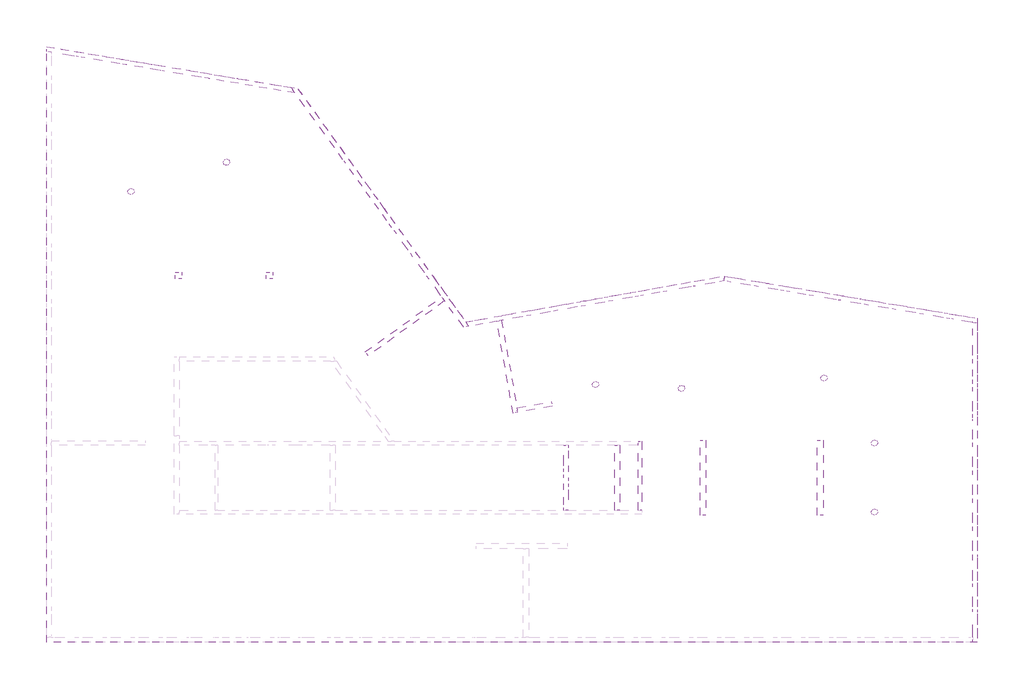
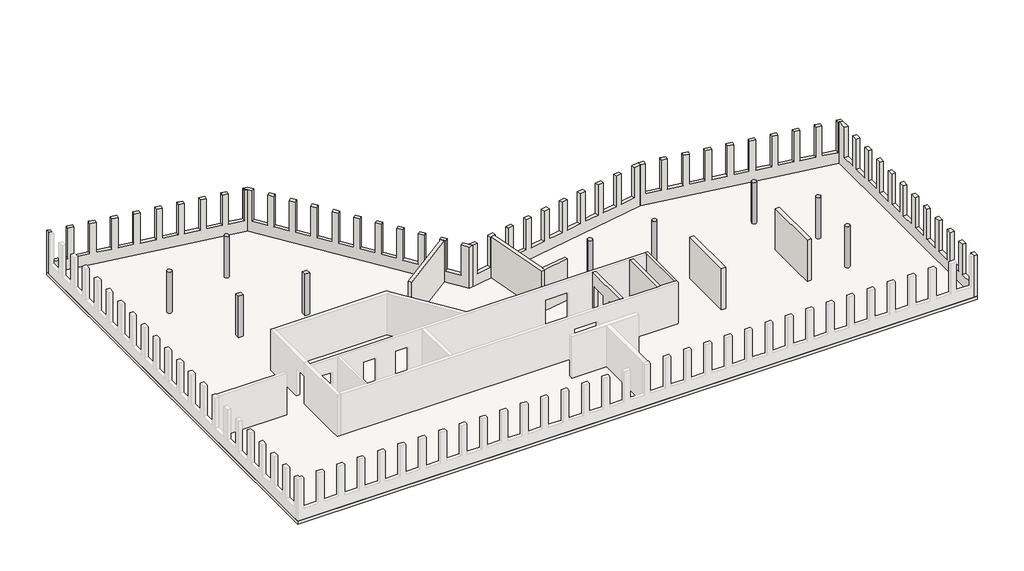
# One storey, part 2 of 2: 13 walls, 9 columns, 1 slab.
"""IFC4 building model written with IfcOpenShell, lengths in millimetres."""

from ifc_helpers import new_model, si_unit, point, frame, frame_2d, origin, place, context, project, spatial, polyline, circle_curve, trimmed, segment, composite_curve, outline, extrude, faceted_brep, element, save

model = new_model("IFC4")

# Units and contexts
model_context = context("Model", 3, world=origin())
ifc_project = project(units=[si_unit("LENGTHUNIT", "METRE", prefix="MILLI")], contexts=[model_context])

# Site, building, storey
site = spatial("IfcSite", under=ifc_project)
building = spatial("IfcBuilding", under=site)
storey = spatial("IfcBuildingStorey", under=building, Name="01_OG_OKFB_3,46", Elevation=3460.0)

# Columns
placement = place(None, origin())
element("IfcColumn", 1, ObjectType="5dki STB-Stützen rund : 5dki Stütze rund ø35cm C40/50", at=placement, inside=storey, context=model_context, shape_type="SweptSolid", body=[
    extrude(outline(composite_curve([segment(trimmed(circle_curve(frame_2d((33961.7583834, 13503.0230367)), 175.0), [point((34136.7583834, 13503.0230367))], [point((33786.7583834, 13503.0230367))], False, "CARTESIAN"), True, "CONTINUOUS"), segment(trimmed(circle_curve(frame_2d((33961.7583834, 13503.0230367)), 175.0), [point((33786.7583834, 13503.0230367))], [point((34136.7583834, 13503.0230367))], False, "CARTESIAN"), True, "CONTINUOUS")], self_intersect=False)), frame((0.0, 0.0, 6770.0), z_axis=(0.0, 0.0, 1.0), x_axis=(1.0, 0.0, 0.0)), (0.0, 0.0, 1.0), 3210.0),
])
element("IfcColumn", 2, ObjectType="5dki STB-Stützen rechteckig : 5dki Stütze recht. 35x35cm C35/45", at=placement, inside=storey, context=model_context, shape_type="SweptSolid", body=[
    extrude(outline(polyline([(7139.9999521, 19742.0124565), (7139.9999521, 19392.0124565), (6789.9999521, 19392.0124565), (6789.9999521, 19742.0124565), (7139.9999521, 19742.0124565)])), frame((0.0, 0.0, 6770.0), z_axis=(0.0, 0.0, 1.0), x_axis=(1.0, 0.0, 0.0)), (0.0, 0.0, 1.0), 3210.0),
])
element("IfcColumn", 3, ObjectType="5dki STB-Stützen rechteckig : 5dki Stütze recht. 35x35cm C35/45", at=placement, inside=storey, context=model_context, shape_type="SweptSolid", body=[
    extrude(outline(polyline([(12021.4450432, 19742.0124565), (12021.4450432, 19392.0124565), (11671.4450432, 19392.0124565), (11671.4450432, 19742.0124565), (12021.4450432, 19742.0124565)])), frame((0.0, 0.0, 6770.0), z_axis=(0.0, 0.0, 1.0), x_axis=(1.0, 0.0, 0.0)), (0.0, 0.0, 1.0), 3210.0),
])
element("IfcColumn", 4, ObjectType="5dki STB-Stützen rund : 5dki Stütze rund ø35cm C40/50", at=placement, inside=storey, context=model_context, shape_type="SweptSolid", body=[
    extrude(outline(composite_curve([segment(trimmed(circle_curve(frame_2d((41616.0718251, 14052.9332427)), 175.0), [point((41791.0718251, 14052.9332427))], [point((41441.0718251, 14052.9332427))], False, "CARTESIAN"), True, "CONTINUOUS"), segment(trimmed(circle_curve(frame_2d((41616.0718251, 14052.9332427)), 175.0), [point((41441.0718251, 14052.9332427))], [point((41791.0718251, 14052.9332427))], False, "CARTESIAN"), True, "CONTINUOUS")], self_intersect=False)), frame((0.0, 0.0, 6770.0), z_axis=(0.0, 0.0, 1.0), x_axis=(1.0, 0.0, 0.0)), (0.0, 0.0, 1.0), 3210.0),
])
element("IfcColumn", 5, ObjectType="5dki STB-Stützen rund : 5dki Stütze rund ø35cm C40/50", at=placement, inside=storey, context=model_context, shape_type="SweptSolid", body=[
    extrude(outline(composite_curve([segment(trimmed(circle_curve(frame_2d((44328.9990923, 10566.8309986)), 175.0), [point((44503.9990923, 10566.8309986))], [point((44153.9990923, 10566.8309986))], False, "CARTESIAN"), True, "CONTINUOUS"), segment(trimmed(circle_curve(frame_2d((44328.9990923, 10566.8309986)), 175.0), [point((44153.9990923, 10566.8309986))], [point((44503.9990923, 10566.8309986))], False, "CARTESIAN"), True, "CONTINUOUS")], self_intersect=False)), frame((0.0, 0.0, 6770.0), z_axis=(0.0, 0.0, 1.0), x_axis=(1.0, 0.0, 0.0)), (0.0, 0.0, 1.0), 3210.0),
])
element("IfcColumn", 6, ObjectType="5dki STB-Stützen rund : 5dki Stütze rund ø35cm C40/50", at=placement, inside=storey, context=model_context, shape_type="SweptSolid", body=[
    extrude(outline(composite_curve([segment(trimmed(circle_curve(frame_2d((44328.9990923, 6852.1619165)), 175.0), [point((44503.9990923, 6852.1619165))], [point((44153.9990923, 6852.1619165))], False, "CARTESIAN"), True, "CONTINUOUS"), segment(trimmed(circle_curve(frame_2d((44328.9990923, 6852.1619165)), 175.0), [point((44153.9990923, 6852.1619165))], [point((44503.9990923, 6852.1619165))], False, "CARTESIAN"), True, "CONTINUOUS")], self_intersect=False)), frame((0.0, 0.0, 6770.0), z_axis=(0.0, 0.0, 1.0), x_axis=(1.0, 0.0, 0.0)), (0.0, 0.0, 1.0), 3210.0),
])
element("IfcColumn", 7, ObjectType="5dki STB-Stützen rund : 5dki Stütze rund ø35cm C40/50", at=placement, inside=storey, context=model_context, shape_type="SweptSolid", body=[
    extrude(outline(composite_curve([segment(trimmed(circle_curve(frame_2d((9535.2710874, 25643.9282611)), 175.0), [point((9710.2710874, 25643.9282611))], [point((9360.2710874, 25643.9282611))], False, "CARTESIAN"), True, "CONTINUOUS"), segment(trimmed(circle_curve(frame_2d((9535.2710874, 25643.9282611)), 175.0), [point((9360.2710874, 25643.9282611))], [point((9710.2710874, 25643.9282611))], False, "CARTESIAN"), True, "CONTINUOUS")], self_intersect=False)), frame((0.0, 0.0, 6770.0), z_axis=(0.0, 0.0, 1.0), x_axis=(1.0, 0.0, 0.0)), (0.0, 0.0, 1.0), 3210.0),
])
element("IfcColumn", 8, ObjectType="5dki STB-Stützen rund : 5dki Stütze rund ø35cm C40/50", at=placement, inside=storey, context=model_context, shape_type="SweptSolid", body=[
    extrude(outline(composite_curve([segment(trimmed(circle_curve(frame_2d((4404.9034618, 24066.2757931)), 175.0), [point((4579.9034618, 24066.2757931))], [point((4229.9034618, 24066.2757931))], False, "CARTESIAN"), True, "CONTINUOUS"), segment(trimmed(circle_curve(frame_2d((4404.9034618, 24066.2757931)), 175.0), [point((4229.9034618, 24066.2757931))], [point((4579.9034618, 24066.2757931))], False, "CARTESIAN"), True, "CONTINUOUS")], self_intersect=False)), frame((0.0, 0.0, 6770.0), z_axis=(0.0, 0.0, 1.0), x_axis=(1.0, 0.0, 0.0)), (0.0, 0.0, 1.0), 3210.0),
])
element("IfcColumn", 9, ObjectType="5dki STB-Stützen rund : 5dki Stütze rund ø35cm C40/50", at=placement, inside=storey, context=model_context, shape_type="SweptSolid", body=[
    extrude(outline(composite_curve([segment(trimmed(circle_curve(frame_2d((29357.7423112, 13702.251654)), 175.0), [point((29532.7423112, 13702.251654))], [point((29182.7423112, 13702.251654))], False, "CARTESIAN"), True, "CONTINUOUS"), segment(trimmed(circle_curve(frame_2d((29357.7423112, 13702.251654)), 175.0), [point((29182.7423112, 13702.251654))], [point((29532.7423112, 13702.251654))], False, "CARTESIAN"), True, "CONTINUOUS")], self_intersect=False)), frame((0.0, 0.0, 6770.0), z_axis=(0.0, 0.0, 1.0), x_axis=(1.0, 0.0, 0.0)), (0.0, 0.0, 1.0), 3210.0),
])

# Slab
element("IfcSlab", 10, ObjectType="5dki Decke Ortbeton 25cm C30/37", at=placement, inside=storey, context=model_context, shape_type="SweptSolid", body=[
    extrude(outline(polyline([(-129.9989953, 31855.7150729), (13359.8955383, 29603.0549033), (22383.5041721, 17069.4128529), (36259.9888873, 19532.5499737), (49863.9990833, 17260.8337794), (49863.9991105, -129.9989509), (-129.9989953, -129.9990284), (-129.9989953, 31855.7150729)]), holes=[polyline([(30391.9999891, 10442.0127433), (27891.9999829, 10442.0127433), (27891.9999829, 6960.0000498), (30391.9999891, 6960.0000498), (30391.9999891, 10442.0127433)]), polyline([(31641.9999382, 10442.0127483), (30641.9999891, 10442.0127483), (30641.9999891, 6960.0000514), (31641.9999382, 6960.0000514), (31641.9999382, 10442.0127483)]), polyline([(8916.9999886, 10442.0127052), (6989.9995723, 10442.0127052), (6989.9995723, 6960.0000232), (8916.9999886, 6960.0000232), (8916.9999886, 10442.0127052)]), polyline([(24127.0004657, 8820.0328918), (16927.0004692, 8820.0328918), (16927.0004692, 7020.033352), (24127.0004657, 7020.033352), (24127.0004657, 8820.0328918)])]), frame((0.0, 0.0, 6520.0), z_axis=(0.0, 0.0, 1.0), x_axis=(1.0, 0.0, 0.0)), (0.0, 0.0, 1.0), 250.0),
])

# Walls
element("IfcWall", 11, ObjectType="5dki Lochfassade 26cm C30/37", at=placement, inside=storey, context=model_context, shape_type="Brep", body=[
    faceted_brep([(12995.7423601, 29663.864375, 6770.0), (13211.4553837, 29364.2425792, 6770.0), (22268.004401, 16784.8468851, 6770.0), (22268.004401, 16784.8468851, 9980.0), (21924.4906268, 17261.9817942, 9980.0), (21924.4906268, 17261.9817942, 7630.0), (21293.4697845, 18138.4592307, 7630.0), (21293.4697845, 18138.4592307, 9980.0), (21048.0727903, 18479.3115671, 9980.0), (21048.0727903, 18479.3115671, 7630.0), (20417.0519481, 19355.7890035, 7630.0), (20417.0519481, 19355.7890035, 9980.0), (20171.6549538, 19696.64134, 9980.0), (20171.6549538, 19696.64134, 7630.0), (19540.6341116, 20573.1187764, 7630.0), (19540.6341116, 20573.1187764, 9980.0), (19295.2371174, 20913.9711128, 9980.0), (19295.2371174, 20913.9711128, 7630.0), (18664.2162751, 21790.4485493, 7630.0), (18664.2162751, 21790.4485493, 9980.0), (18418.8192809, 22131.3008857, 9980.0), (18418.8192809, 22131.3008857, 7630.0), (17787.7984387, 23007.7783222, 7630.0), (17787.7984387, 23007.7783222, 9980.0), (17542.4014445, 23348.6306586, 9980.0), (17542.4014445, 23348.6306586, 7630.0), (16911.3806022, 24225.1080951, 7630.0), (16911.3806022, 24225.1080951, 9980.0), (16665.983608, 24565.9604315, 9980.0), (16665.983608, 24565.9604315, 7630.0), (16034.9627658, 25442.4378679, 7630.0), (16034.9627658, 25442.4378679, 9980.0), (15789.5657715, 25783.2902043, 9980.0), (15789.5657715, 25783.2902043, 7630.0), (15158.5449293, 26659.7676408, 7630.0), (15158.5449293, 26659.7676408, 9980.0), (14913.1479351, 27000.6199772, 9980.0), (14913.1479351, 27000.6199772, 7630.0), (14282.1270928, 27877.0974137, 7630.0), (14282.1270928, 27877.0974137, 9980.0), (14036.7300986, 28217.9497501, 9980.0), (14036.7300986, 28217.9497501, 7630.0), (13405.7092564, 29094.4271866, 7630.0), (13405.7092564, 29094.4271866, 9980.0), (13211.4553837, 29364.2425792, 9980.0), (13028.1664453, 29618.8278609, 9980.0), (13028.1664453, 29618.8278609, 7630.0), (12995.7423601, 29663.864375, 7630.0), (22552.0750732, 16835.2706799, 6770.0), (22383.5041721, 17069.4128529, 6770.0), (13359.8955383, 29603.0549033, 6770.0), (13359.8955383, 29603.0549033, 9980.0), (13616.7130837, 29246.3396115, 9980.0), (13616.7130837, 29246.3396115, 7630.0), (14247.7339259, 28369.8621751, 7630.0), (14247.7339259, 28369.8621751, 9980.0), (14493.1309201, 28029.0098387, 9980.0), (14493.1309201, 28029.0098387, 7630.0), (15124.1517624, 27152.5324022, 7630.0), (15124.1517624, 27152.5324022, 9980.0), (15369.5487566, 26811.6800658, 9980.0), (15369.5487566, 26811.6800658, 7630.0), (16000.5695988, 25935.2026293, 7630.0), (16000.5695988, 25935.2026293, 9980.0), (16245.966593, 25594.3502929, 9980.0), (16245.966593, 25594.3502929, 7630.0), (16876.9874353, 24717.8728564, 7630.0), (16876.9874353, 24717.8728564, 9980.0), (17122.3844295, 24377.02052, 9980.0), (17122.3844295, 24377.02052, 7630.0), (17753.4052718, 23500.5430836, 7630.0), (17753.4052718, 23500.5430836, 9980.0), (17998.802266, 23159.6907472, 9980.0), (17998.802266, 23159.6907472, 7630.0), (18629.8231082, 22283.2133107, 7630.0), (18629.8231082, 22283.2133107, 9980.0), (18875.2201024, 21942.3609743, 9980.0), (18875.2201024, 21942.3609743, 7630.0), (19506.2409447, 21065.8835378, 7630.0), (19506.2409447, 21065.8835378, 9980.0), (19751.6379389, 20725.0312014, 9980.0), (19751.6379389, 20725.0312014, 7630.0), (20382.6587811, 19848.5537649, 7630.0), (20382.6587811, 19848.5537649, 9980.0), (20628.0557754, 19507.7014285, 9980.0), (20628.0557754, 19507.7014285, 7630.0), (21259.0766176, 18631.2239921, 7630.0), (21259.0766176, 18631.2239921, 9980.0), (21504.4736118, 18290.3716557, 9980.0), (21504.4736118, 18290.3716557, 7630.0), (22135.4944541, 17413.8942192, 7630.0), (22135.4944541, 17413.8942192, 9980.0), (22383.5041721, 17069.4128529, 9980.0), (22552.0750732, 16835.2706799, 9980.0), (13034.6033862, 29657.3750221, 9980.0), (13034.6033862, 29657.3750221, 7630.0)], [[[0, 1, 2, 3, 4, 5, 6, 7, 8, 9, 10, 11, 12, 13, 14, 15, 16, 17, 18, 19, 20, 21, 22, 23, 24, 25, 26, 27, 28, 29, 30, 31, 32, 33, 34, 35, 36, 37, 38, 39, 40, 41, 42, 43, 44, 45, 46, 47]], [[48, 49, 50, 51, 52, 53, 54, 55, 56, 57, 58, 59, 60, 61, 62, 63, 64, 65, 66, 67, 68, 69, 70, 71, 72, 73, 74, 75, 76, 77, 78, 79, 80, 81, 82, 83, 84, 85, 86, 87, 88, 89, 90, 91, 92, 93]], [[2, 1, 0, 50, 49, 48]], [[3, 93, 92, 91, 4]], [[52, 51, 94, 45, 44, 43]], [[55, 40, 39, 56]], [[59, 36, 35, 60]], [[63, 32, 31, 64]], [[67, 28, 27, 68]], [[71, 24, 23, 72]], [[75, 20, 19, 76]], [[79, 16, 15, 80]], [[83, 12, 11, 84]], [[87, 8, 7, 88]], [[3, 2, 48, 93]], [[42, 53, 52, 43]], [[54, 41, 40, 55]], [[53, 42, 41, 54]], [[39, 38, 57, 56]], [[37, 36, 59, 58]], [[38, 37, 58, 57]], [[35, 34, 61, 60]], [[33, 32, 63, 62]], [[34, 33, 62, 61]], [[31, 30, 65, 64]], [[29, 28, 67, 66]], [[30, 29, 66, 65]], [[27, 26, 69, 68]], [[25, 24, 71, 70]], [[26, 25, 70, 69]], [[23, 22, 73, 72]], [[21, 20, 75, 74]], [[22, 21, 74, 73]], [[19, 18, 77, 76]], [[17, 16, 79, 78]], [[18, 17, 78, 77]], [[15, 14, 81, 80]], [[13, 12, 83, 82]], [[14, 13, 82, 81]], [[11, 10, 85, 84]], [[9, 8, 87, 86]], [[10, 9, 86, 85]], [[7, 6, 89, 88]], [[5, 4, 91, 90]], [[6, 5, 90, 89]], [[51, 50, 0, 47, 95, 94]], [[95, 46, 45, 94]], [[46, 95, 47]]]),
])
element("IfcWall", 12, ObjectType="5dki Lochfassade 26cm C30/37", at=placement, inside=storey, context=model_context, shape_type="Brep", body=[
    faceted_brep([(27318.6765704, 17681.3634281, 9980.0), (26924.8330267, 17611.4544654, 9980.0), (26924.8330267, 17611.4544654, 7630.0), (25861.4554587, 17422.7002661, 7630.0), (25861.4554587, 17422.7002661, 9980.0), (25447.9197377, 17349.2958553, 9980.0), (25447.9197377, 17349.2958553, 7630.0), (24384.5421697, 17160.541656, 7630.0), (24384.5421697, 17160.541656, 9980.0), (24300.8505369, 17145.6860228, 9980.0), (24054.698322, 17101.9929211, 9980.0), (23971.0064488, 17087.1372452, 9980.0), (23971.0064488, 17087.1372452, 7630.0), (22907.6288807, 16898.3830459, 7630.0), (22907.6288807, 16898.3830459, 9980.0), (22552.0750732, 16835.2706799, 9980.0), (22552.0750732, 16835.2706799, 6770.0), (24054.698322, 17101.9929211, 6770.0), (24300.8505369, 17145.6860228, 6770.0), (36261.33607, 19268.7248546, 6770.0), (36261.33607, 19268.7248546, 9980.0), (35766.6205834, 19180.910678, 9980.0), (35766.6205834, 19180.910678, 7630.0), (34703.2430153, 18992.1564787, 7630.0), (34703.2430153, 18992.1564787, 9980.0), (34289.7072944, 18918.7520679, 9980.0), (34289.7072944, 18918.7520679, 7630.0), (33226.3297263, 18729.9978686, 7630.0), (33226.3297263, 18729.9978686, 9980.0), (32812.7940054, 18656.5934577, 9980.0), (32812.7940054, 18656.5934577, 7630.0), (31749.4164374, 18467.8392585, 7630.0), (31749.4164374, 18467.8392585, 9980.0), (31335.8807164, 18394.4348476, 9980.0), (31335.8807164, 18394.4348476, 7630.0), (30272.5031484, 18205.6806483, 7630.0), (30272.5031484, 18205.6806483, 9980.0), (29858.9674275, 18132.2762375, 9980.0), (29858.9674275, 18132.2762375, 7630.0), (28795.5898594, 17943.5220382, 7630.0), (28795.5898594, 17943.5220382, 9980.0), (28382.0541385, 17870.1176274, 9980.0), (28382.0541385, 17870.1176274, 7630.0), (27318.6765704, 17681.3634281, 7630.0), (26879.392201, 17867.4527688, 7630.0), (26879.392201, 17867.4527688, 9980.0), (27273.2357447, 17937.3617315, 9980.0), (27273.2357447, 17937.3617315, 7630.0), (28336.6133127, 18126.1159308, 7630.0), (28336.6133127, 18126.1159308, 9980.0), (28750.1490337, 18199.5203416, 9980.0), (28750.1490337, 18199.5203416, 7630.0), (29813.5266017, 18388.2745409, 7630.0), (29813.5266017, 18388.2745409, 9980.0), (30227.0623226, 18461.6789518, 9980.0), (30227.0623226, 18461.6789518, 7630.0), (31290.4398907, 18650.433151, 7630.0), (31290.4398907, 18650.433151, 9980.0), (31703.9756116, 18723.8375619, 9980.0), (31703.9756116, 18723.8375619, 7630.0), (32767.3531797, 18912.5917612, 7630.0), (32767.3531797, 18912.5917612, 9980.0), (33180.8889006, 18985.996172, 9980.0), (33180.8889006, 18985.996172, 7630.0), (34244.2664686, 19174.7503713, 7630.0), (34244.2664686, 19174.7503713, 9980.0), (34657.8021895, 19248.1547821, 9980.0), (34657.8021895, 19248.1547821, 7630.0), (35721.1797576, 19436.9089814, 7630.0), (35721.1797576, 19436.9089814, 9980.0), (36259.9888873, 19532.5499737, 9980.0), (36259.9888873, 19532.5499737, 6770.0), (22383.5041721, 17069.4128529, 6770.0), (22383.5041721, 17069.4128529, 9980.0), (22862.188055, 17154.3813493, 9980.0), (22862.188055, 17154.3813493, 7630.0), (23925.565623, 17343.1355486, 7630.0), (23925.565623, 17343.1355486, 9980.0), (24339.1013439, 17416.5399594, 9980.0), (24339.1013439, 17416.5399594, 7630.0), (25402.478912, 17605.2941587, 7630.0), (25402.478912, 17605.2941587, 9980.0), (25816.0146329, 17678.6985695, 9980.0), (25816.0146329, 17678.6985695, 7630.0)], [[[0, 1, 2, 3, 4, 5, 6, 7, 8, 9, 10, 11, 12, 13, 14, 15, 16, 17, 18, 19, 20, 21, 22, 23, 24, 25, 26, 27, 28, 29, 30, 31, 32, 33, 34, 35, 36, 37, 38, 39, 40, 41, 42, 43]], [[44, 45, 46, 47, 48, 49, 50, 51, 52, 53, 54, 55, 56, 57, 58, 59, 60, 61, 62, 63, 64, 65, 66, 67, 68, 69, 70, 71, 72, 73, 74, 75, 76, 77, 78, 79, 80, 81, 82, 83]], [[19, 18, 17, 16, 72, 71]], [[74, 73, 15, 14]], [[50, 49, 41, 40]], [[37, 36, 54, 53]], [[58, 57, 33, 32]], [[29, 28, 62, 61]], [[21, 20, 70, 69]], [[25, 24, 66, 65]], [[78, 77, 11, 10, 9, 8]], [[82, 81, 5, 4]], [[46, 45, 1, 0]], [[16, 15, 73, 72]], [[20, 19, 71, 70]], [[14, 13, 75, 74]], [[12, 11, 77, 76]], [[13, 12, 76, 75]], [[49, 48, 42, 41]], [[47, 46, 0, 43]], [[48, 47, 43, 42]], [[40, 39, 51, 50]], [[38, 37, 53, 52]], [[39, 38, 52, 51]], [[57, 56, 34, 33]], [[55, 54, 36, 35]], [[56, 55, 35, 34]], [[32, 31, 59, 58]], [[30, 29, 61, 60]], [[31, 30, 60, 59]], [[65, 64, 26, 25]], [[63, 62, 28, 27]], [[64, 63, 27, 26]], [[69, 68, 22, 21]], [[67, 66, 24, 23]], [[68, 67, 23, 22]], [[8, 7, 79, 78]], [[6, 5, 81, 80]], [[7, 6, 80, 79]], [[4, 3, 83, 82]], [[2, 1, 45, 44]], [[3, 2, 44, 83]]]),
])
element("IfcWall", 13, ObjectType="5dki Lochfassade 26cm C30/37", at=placement, inside=storey, context=model_context, shape_type="Brep", body=[
    faceted_brep([(49863.9990837, 16997.2336245, 9980.0), (49603.9990837, 17040.6506907, 9980.0), (49507.8677901, 17056.7035319, 9980.0), (49507.8677901, 17056.7035319, 7630.0), (48442.6180365, 17234.5882205, 7630.0), (48442.6180365, 17234.5882205, 9980.0), (48028.3542434, 17303.7655993, 9980.0), (48028.3542434, 17303.7655993, 7630.0), (46963.1044898, 17481.6502878, 7630.0), (46963.1044898, 17481.6502878, 9980.0), (46548.8406967, 17550.8276667, 9980.0), (46548.8406967, 17550.8276667, 7630.0), (45483.5909431, 17728.7123552, 7630.0), (45483.5909431, 17728.7123552, 9980.0), (45069.32715, 17797.8897341, 9980.0), (45069.32715, 17797.8897341, 7630.0), (44004.0773964, 17975.7744226, 7630.0), (44004.0773964, 17975.7744226, 9980.0), (43589.8136033, 18044.9518015, 9980.0), (43589.8136033, 18044.9518015, 7630.0), (42524.5638497, 18222.83649, 7630.0), (42524.5638497, 18222.83649, 9980.0), (42110.3000566, 18292.0138689, 9980.0), (42110.3000566, 18292.0138689, 7630.0), (41045.050303, 18469.8985574, 7630.0), (41045.050303, 18469.8985574, 9980.0), (40630.7865099, 18539.0759362, 9980.0), (40630.7865099, 18539.0759362, 7630.0), (39565.5367563, 18716.9606248, 7630.0), (39565.5367563, 18716.9606248, 9980.0), (39151.2729632, 18786.1380036, 9980.0), (39151.2729632, 18786.1380036, 7630.0), (38086.0232096, 18964.0226921, 7630.0), (38086.0232096, 18964.0226921, 9980.0), (37671.7594165, 19033.200071, 9980.0), (37671.7594165, 19033.200071, 7630.0), (36606.5096629, 19211.0847595, 7630.0), (36606.5096629, 19211.0847595, 9980.0), (36261.33607, 19268.7248546, 9980.0), (36261.33607, 19268.7248546, 6770.0), (49603.9990837, 17040.6506907, 6770.0), (49863.9990837, 16997.2336245, 6770.0), (49550.6918818, 17313.1525467, 7630.0), (49550.6918818, 17313.1525467, 9980.0), (49863.9990833, 17260.8337794, 9980.0), (49863.9990833, 17260.8337794, 6770.0), (36259.9888873, 19532.5499737, 6770.0), (36259.9888873, 19532.5499737, 9980.0), (36649.3337546, 19467.5337743, 9980.0), (36649.3337546, 19467.5337743, 7630.0), (37714.5835082, 19289.6490858, 7630.0), (37714.5835082, 19289.6490858, 9980.0), (38128.8473013, 19220.4717069, 9980.0), (38128.8473013, 19220.4717069, 7630.0), (39194.0970549, 19042.5870184, 7630.0), (39194.0970549, 19042.5870184, 9980.0), (39608.360848, 18973.4096395, 9980.0), (39608.360848, 18973.4096395, 7630.0), (40673.6106016, 18795.524951, 7630.0), (40673.6106016, 18795.524951, 9980.0), (41087.8743947, 18726.3475721, 9980.0), (41087.8743947, 18726.3475721, 7630.0), (42153.1241483, 18548.4628836, 7630.0), (42153.1241483, 18548.4628836, 9980.0), (42567.3879414, 18479.2855048, 9980.0), (42567.3879414, 18479.2855048, 7630.0), (43632.637695, 18301.4008162, 7630.0), (43632.637695, 18301.4008162, 9980.0), (44046.9014881, 18232.2234374, 9980.0), (44046.9014881, 18232.2234374, 7630.0), (45112.1512417, 18054.3387489, 7630.0), (45112.1512417, 18054.3387489, 9980.0), (45526.4150348, 17985.16137, 9980.0), (45526.4150348, 17985.16137, 7630.0), (46591.6647884, 17807.2766815, 7630.0), (46591.6647884, 17807.2766815, 9980.0), (47005.9285815, 17738.0993026, 9980.0), (47005.9285815, 17738.0993026, 7630.0), (48071.1783351, 17560.2146141, 7630.0), (48071.1783351, 17560.2146141, 9980.0), (48485.4421282, 17491.0372352, 9980.0), (48485.4421282, 17491.0372352, 7630.0)], [[[0, 1, 2, 3, 4, 5, 6, 7, 8, 9, 10, 11, 12, 13, 14, 15, 16, 17, 18, 19, 20, 21, 22, 23, 24, 25, 26, 27, 28, 29, 30, 31, 32, 33, 34, 35, 36, 37, 38, 39, 40, 41]], [[42, 43, 44, 45, 46, 47, 48, 49, 50, 51, 52, 53, 54, 55, 56, 57, 58, 59, 60, 61, 62, 63, 64, 65, 66, 67, 68, 69, 70, 71, 72, 73, 74, 75, 76, 77, 78, 79, 80, 81]], [[41, 40, 39, 46, 45]], [[48, 47, 38, 37]], [[52, 51, 34, 33]], [[56, 55, 30, 29]], [[60, 59, 26, 25]], [[64, 63, 22, 21]], [[68, 67, 18, 17]], [[72, 71, 14, 13]], [[76, 75, 10, 9]], [[80, 79, 6, 5]], [[44, 43, 2, 1, 0]], [[39, 38, 47, 46]], [[0, 41, 45, 44]], [[37, 36, 49, 48]], [[35, 34, 51, 50]], [[36, 35, 50, 49]], [[33, 32, 53, 52]], [[31, 30, 55, 54]], [[32, 31, 54, 53]], [[29, 28, 57, 56]], [[27, 26, 59, 58]], [[28, 27, 58, 57]], [[25, 24, 61, 60]], [[23, 22, 63, 62]], [[24, 23, 62, 61]], [[21, 20, 65, 64]], [[19, 18, 67, 66]], [[20, 19, 66, 65]], [[17, 16, 69, 68]], [[15, 14, 71, 70]], [[16, 15, 70, 69]], [[13, 12, 73, 72]], [[11, 10, 75, 74]], [[12, 11, 74, 73]], [[9, 8, 77, 76]], [[7, 6, 79, 78]], [[8, 7, 78, 77]], [[5, 4, 81, 80]], [[3, 2, 43, 42]], [[4, 3, 42, 81]]]),
])
element("IfcWall", 14, ObjectType="5dki Lochfassade 26cm C30/37", at=placement, inside=storey, context=model_context, shape_type="Brep", body=[
    faceted_brep([(49603.9991105, -129.9989514, 9980.0), (49603.9991101, 130.0010486, 9980.0), (49603.9991099, 277.0124979, 9980.0), (49603.9991099, 277.0124979, 7630.0), (49603.9991082, 1357.0124979, 7630.0), (49603.9991082, 1357.0124979, 9980.0), (49603.9991075, 1777.0124979, 9980.0), (49603.9991075, 1777.0124979, 7630.0), (49603.9991058, 2857.0124979, 7630.0), (49603.9991058, 2857.0124979, 9980.0), (49603.9991052, 3277.0124979, 9980.0), (49603.9991052, 3277.0124979, 7630.0), (49603.9991035, 4357.0124979, 7630.0), (49603.9991035, 4357.0124979, 9980.0), (49603.9991028, 4777.0124979, 9980.0), (49603.9991028, 4777.0124979, 7630.0), (49603.9991011, 5857.0124979, 7630.0), (49603.9991011, 5857.0124979, 9980.0), (49603.9991005, 6277.0124979, 9980.0), (49603.9991005, 6277.0124979, 7630.0), (49603.9990988, 7357.0124979, 7630.0), (49603.9990988, 7357.0124979, 9980.0), (49603.9990981, 7777.0124979, 9980.0), (49603.9990981, 7777.0124979, 7630.0), (49603.9990964, 8857.0124979, 7630.0), (49603.9990964, 8857.0124979, 9980.0), (49603.9990958, 9277.0124979, 9980.0), (49603.9990958, 9277.0124979, 7630.0), (49603.9990941, 10357.0124979, 7630.0), (49603.9990941, 10357.0124979, 9980.0), (49603.9990934, 10777.0124979, 9980.0), (49603.9990934, 10777.0124979, 7630.0), (49603.9990918, 11857.0124979, 7630.0), (49603.9990918, 11857.0124979, 9980.0), (49603.9990911, 12277.0124979, 9980.0), (49603.9990911, 12277.0124979, 7630.0), (49603.9990894, 13357.0124979, 7630.0), (49603.9990894, 13357.0124979, 9980.0), (49603.9990888, 13777.0124979, 9980.0), (49603.9990888, 13777.0124979, 7630.0), (49603.9990871, 14857.0124979, 7630.0), (49603.9990871, 14857.0124979, 9980.0), (49603.9990864, 15277.0124979, 9980.0), (49603.9990864, 15277.0124979, 7630.0), (49603.9990847, 16357.0124979, 7630.0), (49603.9990847, 16357.0124979, 9980.0), (49603.9990837, 17040.6506907, 9980.0), (49603.9990837, 17040.6506907, 6770.0), (49603.9991101, 130.0010486, 6770.0), (49603.9991105, -129.9989514, 6770.0), (49863.9991099, 277.0124983, 7630.0), (49863.9991099, 277.0124983, 9980.0), (49863.9991105, -129.9989509, 9980.0), (49863.9991105, -129.9989509, 6770.0), (49863.9990837, 16997.2336245, 6770.0), (49863.9990837, 16997.2336245, 9980.0), (49863.9990847, 16357.0124983, 9980.0), (49863.9990847, 16357.0124983, 7630.0), (49863.9990864, 15277.0124983, 7630.0), (49863.9990864, 15277.0124983, 9980.0), (49863.9990871, 14857.0124983, 9980.0), (49863.9990871, 14857.0124983, 7630.0), (49863.9990888, 13777.0124983, 7630.0), (49863.9990888, 13777.0124983, 9980.0), (49863.9990894, 13357.0124983, 9980.0), (49863.9990894, 13357.0124983, 7630.0), (49863.9990911, 12277.0124983, 7630.0), (49863.9990911, 12277.0124983, 9980.0), (49863.9990918, 11857.0124983, 9980.0), (49863.9990918, 11857.0124983, 7630.0), (49863.9990934, 10777.0124983, 7630.0), (49863.9990934, 10777.0124983, 9980.0), (49863.9990941, 10357.0124983, 9980.0), (49863.9990941, 10357.0124983, 7630.0), (49863.9990958, 9277.0124983, 7630.0), (49863.9990958, 9277.0124983, 9980.0), (49863.9990964, 8857.0124983, 9980.0), (49863.9990964, 8857.0124983, 7630.0), (49863.9990981, 7777.0124983, 7630.0), (49863.9990981, 7777.0124983, 9980.0), (49863.9990988, 7357.0124983, 9980.0), (49863.9990988, 7357.0124983, 7630.0), (49863.9991005, 6277.0124983, 7630.0), (49863.9991005, 6277.0124983, 9980.0), (49863.9991011, 5857.0124983, 9980.0), (49863.9991011, 5857.0124983, 7630.0), (49863.9991028, 4777.0124983, 7630.0), (49863.9991028, 4777.0124983, 9980.0), (49863.9991035, 4357.0124983, 9980.0), (49863.9991035, 4357.0124983, 7630.0), (49863.9991052, 3277.0124983, 7630.0), (49863.9991052, 3277.0124983, 9980.0), (49863.9991058, 2857.0124983, 9980.0), (49863.9991058, 2857.0124983, 7630.0), (49863.9991075, 1777.0124983, 7630.0), (49863.9991075, 1777.0124983, 9980.0), (49863.9991082, 1357.0124983, 9980.0), (49863.9991082, 1357.0124983, 7630.0)], [[[0, 1, 2, 3, 4, 5, 6, 7, 8, 9, 10, 11, 12, 13, 14, 15, 16, 17, 18, 19, 20, 21, 22, 23, 24, 25, 26, 27, 28, 29, 30, 31, 32, 33, 34, 35, 36, 37, 38, 39, 40, 41, 42, 43, 44, 45, 46, 47, 48, 49]], [[50, 51, 52, 53, 54, 55, 56, 57, 58, 59, 60, 61, 62, 63, 64, 65, 66, 67, 68, 69, 70, 71, 72, 73, 74, 75, 76, 77, 78, 79, 80, 81, 82, 83, 84, 85, 86, 87, 88, 89, 90, 91, 92, 93, 94, 95, 96, 97]], [[49, 48, 47, 54, 53]], [[55, 46, 45, 56]], [[42, 41, 60, 59]], [[38, 37, 64, 63]], [[34, 33, 68, 67]], [[30, 29, 72, 71]], [[26, 25, 76, 75]], [[22, 21, 80, 79]], [[18, 17, 84, 83]], [[14, 13, 88, 87]], [[10, 9, 92, 91]], [[96, 95, 6, 5]], [[52, 51, 2, 1, 0]], [[47, 46, 55, 54]], [[0, 49, 53, 52]], [[58, 43, 42, 59]], [[44, 57, 56, 45]], [[43, 58, 57, 44]], [[63, 62, 39, 38]], [[61, 60, 41, 40]], [[62, 61, 40, 39]], [[67, 66, 35, 34]], [[65, 64, 37, 36]], [[66, 65, 36, 35]], [[71, 70, 31, 30]], [[69, 68, 33, 32]], [[70, 69, 32, 31]], [[75, 74, 27, 26]], [[73, 72, 29, 28]], [[74, 73, 28, 27]], [[79, 78, 23, 22]], [[77, 76, 25, 24]], [[78, 77, 24, 23]], [[83, 82, 19, 18]], [[81, 80, 21, 20]], [[82, 81, 20, 19]], [[87, 86, 15, 14]], [[85, 84, 17, 16]], [[86, 85, 16, 15]], [[91, 90, 11, 10]], [[89, 88, 13, 12]], [[90, 89, 12, 11]], [[95, 94, 7, 6]], [[93, 92, 9, 8]], [[94, 93, 8, 7]], [[5, 4, 97, 96]], [[3, 2, 51, 50]], [[4, 3, 50, 97]]]),
])
element("IfcWall", 15, ObjectType="5dki STB-Wand Kern 25cm C30/37", at=placement, inside=storey, context=model_context, shape_type="SweptSolid", body=[
    extrude(outline(polyline([(30641.9999891, 10442.0127483), (30641.9999891, 6960.0000501), (30391.9999891, 6960.0000498), (30391.9999891, 10442.0127479), (30641.9999891, 10442.0127483)])), frame((0.0, 0.0, 6770.0), z_axis=(0.0, 0.0, 1.0), x_axis=(1.0, 0.0, 0.0)), (0.0, 0.0, 1.0), 3210.0),
])
element("IfcWall", 16, ObjectType="5dki STB-Wand Kern 25cm C30/37", at=placement, inside=storey, context=model_context, shape_type="SweptSolid", body=[
    extrude(outline(polyline([(3482.0126944, -3210.0), (-2.1e-06, -3210.0), (-2.1e-06, 0.0), (279.9681323, 0.0), (279.9681323, -2260.0), (1414.9681323, -2260.0), (1414.9681323, 0.0), (2067.1995869, 0.0), (2067.1995869, -2260.0), (3202.1995869, -2260.0), (3202.1995869, 0.0), (3482.0126944, 0.0), (3482.0126944, -3210.0)])), frame((27641.9999829, 10442.0127408, 6770.0), z_axis=(1.0, 1.6300916066412081e-09, 0.0), x_axis=(1.6300916066412081e-09, -1.0, 0.0)), (0.0, 0.0, 1.0), 250.0),
])
element("IfcWall", 17, ObjectType="5dki STB-Wand Kern 20cm C35/45", at=placement, inside=storey, context=model_context, shape_type="Brep", body=[
    faceted_brep([(31641.9999912, 10662.0127502, 6770.0), (31641.9999881, 10442.0127502, 6770.0), (31641.9999382, 6960.0000514, 6770.0), (31641.9999382, 6960.0000514, 9980.0), (31641.9999881, 10442.0127502, 9980.0), (31641.9999912, 10662.0127502, 9980.0), (31841.9999912, 10662.0127505, 6770.0), (31841.9999912, 10662.0127505, 9980.0), (31841.9999382, 6960.0000516, 9980.0), (31841.9999382, 6960.0000516, 6770.0)], [[[0, 1, 2, 3, 4, 5]], [[6, 7, 8, 9]], [[2, 1, 0, 6, 9]], [[5, 4, 3, 8, 7]], [[0, 5, 7, 6]], [[3, 2, 9, 8]]]),
])
element("IfcWall", 18, ObjectType="5dki Lochfassade 26cm C30/37", at=placement, inside=storey, context=model_context, shape_type="Brep", body=[
    faceted_brep([(8967.5024476, 30072.9348316, 7630.0), (8967.5024476, 30072.9348316, 9980.0), (8553.2386546, 30142.1122105, 9980.0), (8553.2386546, 30142.1122105, 7630.0), (7487.988901, 30319.9968993, 7630.0), (7487.988901, 30319.9968993, 9980.0), (7073.7251079, 30389.1742783, 9980.0), (7073.7251079, 30389.1742783, 7630.0), (6008.4753544, 30567.058967, 7630.0), (6008.4753544, 30567.058967, 9980.0), (5594.2115613, 30636.236346, 9980.0), (5594.2115613, 30636.236346, 7630.0), (4528.9618077, 30814.1210348, 7630.0), (4528.9618077, 30814.1210348, 9980.0), (4114.6980147, 30883.2984137, 9980.0), (4114.6980147, 30883.2984137, 7630.0), (3049.4482611, 31061.1831025, 7630.0), (3049.4482611, 31061.1831025, 9980.0), (2635.184468, 31130.3604815, 9980.0), (2635.184468, 31130.3604815, 7630.0), (1569.9347144, 31308.2451702, 7630.0), (1569.9347144, 31308.2451702, 9980.0), (1155.6709214, 31377.4225492, 9980.0), (1155.6709214, 31377.4225492, 7630.0), (90.4211678, 31555.307238, 7630.0), (90.4211678, 31555.307238, 9980.0), (-129.9989953, 31592.114918, 9980.0), (-129.9989953, 31592.114918, 6770.0), (130.0010047, 31548.6978518, 6770.0), (13211.4553837, 29364.2425792, 6770.0), (13211.4553837, 29364.2425792, 9980.0), (12991.7792945, 29400.9260074, 9980.0), (12991.7792945, 29400.9260074, 7630.0), (11926.5295409, 29578.8106961, 7630.0), (11926.5295409, 29578.8106961, 9980.0), (11512.2657479, 29647.9880751, 9980.0), (11512.2657479, 29647.9880751, 7630.0), (10447.0159943, 29825.8727639, 7630.0), (10447.0159943, 29825.8727639, 9980.0), (10032.7522012, 29895.0501428, 9980.0), (10032.7522012, 29895.0501428, 7630.0), (8596.0627463, 30398.5612253, 9980.0), (9010.3265394, 30329.3838463, 9980.0), (9010.3265394, 30329.3838463, 7630.0), (10075.576293, 30151.4991576, 7630.0), (10075.576293, 30151.4991576, 9980.0), (10489.840086, 30082.3217786, 9980.0), (10489.840086, 30082.3217786, 7630.0), (11555.0898396, 29904.4370898, 7630.0), (11555.0898396, 29904.4370898, 9980.0), (11969.3536327, 29835.2597109, 9980.0), (11969.3536327, 29835.2597109, 7630.0), (12995.7423601, 29663.864375, 7630.0), (12995.7423601, 29663.864375, 6770.0), (-129.9989953, 31855.7150729, 6770.0), (-129.9989953, 31855.7150729, 9980.0), (133.2452595, 31811.7562527, 9980.0), (133.2452595, 31811.7562527, 7630.0), (1198.4950131, 31633.8715639, 7630.0), (1198.4950131, 31633.8715639, 9980.0), (1612.7588062, 31564.694185, 9980.0), (1612.7588062, 31564.694185, 7630.0), (2678.0085598, 31386.8094962, 7630.0), (2678.0085598, 31386.8094962, 9980.0), (3092.2723528, 31317.6321172, 9980.0), (3092.2723528, 31317.6321172, 7630.0), (4157.5221064, 31139.7474285, 7630.0), (4157.5221064, 31139.7474285, 9980.0), (4571.7858995, 31070.5700495, 9980.0), (4571.7858995, 31070.5700495, 7630.0), (5637.035653, 30892.6853608, 7630.0), (5637.035653, 30892.6853608, 9980.0), (6051.2994461, 30823.5079818, 9980.0), (6051.2994461, 30823.5079818, 7630.0), (7116.5491997, 30645.623293, 7630.0), (7116.5491997, 30645.623293, 9980.0), (7530.8129927, 30576.4459141, 9980.0), (7530.8129927, 30576.4459141, 7630.0), (8596.0627463, 30398.5612253, 7630.0), (13028.1664453, 29618.8278609, 9980.0), (13028.1664453, 29618.8278609, 7630.0)], [[[0, 1, 2, 3, 4, 5, 6, 7, 8, 9, 10, 11, 12, 13, 14, 15, 16, 17, 18, 19, 20, 21, 22, 23, 24, 25, 26, 27, 28, 29, 30, 31, 32, 33, 34, 35, 36, 37, 38, 39, 40]], [[41, 42, 43, 44, 45, 46, 47, 48, 49, 50, 51, 52, 53, 54, 55, 56, 57, 58, 59, 60, 61, 62, 63, 64, 65, 66, 67, 68, 69, 70, 71, 72, 73, 74, 75, 76, 77, 78]], [[29, 28, 27, 54, 53]], [[49, 35, 34, 50]], [[22, 21, 60, 59]], [[18, 17, 64, 63]], [[14, 13, 68, 67]], [[10, 9, 72, 71]], [[6, 5, 76, 75]], [[39, 38, 46, 45]], [[2, 1, 42, 41]], [[31, 30, 79]], [[55, 26, 25, 56]], [[37, 47, 46, 38]], [[48, 36, 35, 49]], [[47, 37, 36, 48]], [[58, 23, 22, 59]], [[24, 57, 56, 25]], [[23, 58, 57, 24]], [[63, 62, 19, 18]], [[61, 60, 21, 20]], [[62, 61, 20, 19]], [[67, 66, 15, 14]], [[65, 64, 17, 16]], [[66, 65, 16, 15]], [[71, 70, 11, 10]], [[69, 68, 13, 12]], [[70, 69, 12, 11]], [[75, 74, 7, 6]], [[73, 72, 9, 8]], [[74, 73, 8, 7]], [[41, 78, 3, 2]], [[77, 76, 5, 4]], [[78, 77, 4, 3]], [[45, 44, 40, 39]], [[43, 42, 1, 0]], [[44, 43, 0, 40]], [[30, 29, 53, 52, 80, 79]], [[33, 51, 50, 34]], [[80, 32, 31, 79]], [[51, 33, 32, 80, 52]], [[27, 26, 55, 54]]]),
])
element("IfcWall", 19, ObjectType="5dki STB-Wand 25cm C30/37", at=placement, inside=storey, context=model_context, shape_type="SweptSolid", body=[
    extrude(outline(polyline([(16994.6178661, 15452.6713643), (21084.845921, 18397.4352698), (21230.9155592, 18194.5469734), (17140.6875043, 15249.783068), (16994.6178661, 15452.6713643)])), frame((0.0, 0.0, 6770.0), z_axis=(0.0, 0.0, 1.0), x_axis=(1.0, 0.0, 0.0)), (0.0, 0.0, 1.0), 3210.0),
])
element("IfcWall", 20, ObjectType="5dki STB-Wand 25cm C30/37", at=placement, inside=storey, context=model_context, shape_type="Brep", body=[
    faceted_brep([(24054.698322, 17101.9929211, 6770.0), (24930.952116, 12165.4742089, 6770.0), (24930.952116, 12165.4742089, 9980.0), (24054.698322, 17101.9929211, 9980.0), (24300.8505369, 17145.6860228, 6770.0), (24300.8505369, 17145.6860228, 9980.0), (25133.4112296, 12455.3195251, 9980.0), (25177.1043309, 12209.1673103, 9980.0), (25177.1043309, 12209.1673103, 6770.0), (25133.4112296, 12455.3195251, 6770.0)], [[[0, 1, 2, 3]], [[4, 5, 6, 7, 8, 9]], [[1, 0, 4, 9, 8]], [[3, 2, 7, 6, 5]], [[0, 3, 5, 4]], [[2, 1, 8, 7]]]),
])
element("IfcWall", 21, ObjectType="5dki STB-Wand 25cm C30/37", at=placement, inside=storey, context=model_context, shape_type="SweptSolid", body=[
    extrude(outline(polyline([(27026.4023238, 12537.4258416), (25177.1043309, 12209.1673103), (25133.4112296, 12455.3195251), (26982.7092225, 12783.5780565), (27026.4023238, 12537.4258416)])), frame((0.0, 0.0, 6770.0), z_axis=(0.0, 0.0, 1.0), x_axis=(1.0, 0.0, 0.0)), (0.0, 0.0, 1.0), 3210.0),
])
element("IfcWall", 22, ObjectType="5dki STB-Wand 30cm C30/37", at=placement, inside=storey, context=model_context, shape_type="SweptSolid", body=[
    extrude(outline(polyline([(34969.9990839, 6680.0000532), (34969.9990776, 10702.0125181), (35269.9990776, 10702.0125186), (35269.9990839, 6680.0000537), (34969.9990839, 6680.0000532)])), frame((0.0, 0.0, 6770.0), z_axis=(0.0, 0.0, 1.0), x_axis=(1.0, 0.0, 0.0)), (0.0, 0.0, 1.0), 3210.0),
])
element("IfcWall", 23, ObjectType="5dki STB-Wand 30cm C30/37", at=placement, inside=storey, context=model_context, shape_type="SweptSolid", body=[
    extrude(outline(polyline([(41269.9990703, 6680.000074), (41269.9990703, 10722.0122605), (41569.9990703, 10722.0122605), (41569.9990703, 6680.000074), (41269.9990703, 6680.000074)])), frame((0.0, 0.0, 6770.0), z_axis=(0.0, 0.0, 1.0), x_axis=(1.0, 0.0, 0.0)), (0.0, 0.0, 1.0), 3210.0),
])

save(model, "model.ifc")

# Revit data of these elements
# Type "5dki STB-Stützen rund : 5dki Stütze rund ø35cm C40/50"
#   cpiFitMatchKey = "5D-KI-STB-OB-ST-RUN"
#   cpiComponentType = "Column"
#   5d Materialgüte = "C40/50"
#   Radius = 0.175 m
#   Durchmesser = 0.350 m
#   5dki Bewehrung Stab kg pro m3 = 0
#   5dki Sichtbeton SB3/SB4 [instance default] = no
#   Structural Material = 5d Beton - Stahlbeton
#   Assembly Code = ""
# Type "5dki STB-Stützen rechteckig : 5dki Stütze recht. 35x35cm C35/45"
#   cpiFitMatchKey = "5D-KI-STB-OB-ST-REC"
#   cpiComponentType = "Column"
#   5d Materialgüte = "C35/45"
#   Tiefe = 0.350 m
#   Breite = 0.350 m
#   5dki Bewehrung Stab kg pro m3 = 0
#   5dki Sichtbeton SB3/SB4 [instance default] = no
#   Structural Material = 5d Beton - Stahlbeton
#   Assembly Code = ""
# Type "5dki Decke Ortbeton 25cm C30/37"
#   cpiComponentType = "Slab"
#   cpiFitMatchKey = "5D-KI-STB-OB-DE"
#   5d Materialgüte = "C30/37"
#   Function = 0
#   5dki WU = no
#   Layers, outside or top first: 0.250 m "5d Beton - Stahlbeton" (function 1)
# Type "5dki Lochfassade 26cm C30/37"
#   Type Comments = ""
#   Description = ""
#   cpiComponentType = "Wall"
#   cpiFitMatchKey = "5D-KI-STB-OB-W-LF"
#   5d Materialgüte = "C35/45"
#   Filter Tragend / Nichttragend = yes
#   5dki WU = no
#   Layers, outside or top first: 0.260 m "5d Beton - Stahlbeton" (function 1)
# Type "5dki STB-Wand Kern 25cm C30/37"
#   Type Comments = ""
#   Description = ""
#   cpiComponentType = "Wall"
#   cpiFitMatchKey = "5D-KI-STB-OB-W-K"
#   5d Materialgüte = "C30/37"
#   Filter Tragend / Nichttragend = yes
#   5dki WU = no
#   Layers, outside or top first: 0.250 m "5d Beton - Stahlbeton" (function 1)
# Type "5dki STB-Wand Kern 20cm C35/45"
#   Type Comments = ""
#   Description = ""
#   cpiComponentType = "Wall"
#   cpiFitMatchKey = "5D-KI-STB-OB-W-K"
#   5d Materialgüte = "C35/45"
#   Filter Tragend / Nichttragend = yes
#   5dki WU = no
#   Layers, outside or top first: 0.200 m "5d Beton - Stahlbeton" (function 1)
# Type "5dki STB-Wand 25cm C30/37"
#   Type Comments = ""
#   Description = ""
#   cpiComponentType = "Wall"
#   cpiFitMatchKey = "5D-KI-STB-OB-W"
#   5d Materialgüte = "C30/37"
#   Filter Tragend / Nichttragend = yes
#   5dki WU = no
#   Layers, outside or top first: 0.250 m "5d Beton - Stahlbeton" (function 1)
# Type "5dki STB-Wand 30cm C30/37"
#   Type Comments = ""
#   Description = ""
#   cpiComponentType = "Wall"
#   cpiFitMatchKey = "5D-KI-STB-OB-W"
#   5d Materialgüte = "C30/37"
#   Filter Tragend / Nichttragend = yes
#   5dki WU = no
#   Layers, outside or top first: 0.300 m "5d Beton - Stahlbeton" (function 1)
# Elements 1, 9 (IfcColumn, "5dki STB-Stützen rund : 5dki Stütze rund ø35cm C40/50")
#   Comments = ""
#   000_080_030_Geschoß = "02_OG"
#   5dki Sichtbeton SB3/SB4 = no
#   Phase Created = Neu
#   Materials on its faces: "5d Beton - Stahlbeton"
# Element 2 (IfcColumn, "5dki STB-Stützen rechteckig : 5dki Stütze recht. 35x35cm C35/45")
#   Comments = ""
#   000_080_030_Geschoß = "02_OG"
#   5dki Sichtbeton SB3/SB4 = no
#   Phase Created = Neu
#   Materials on its faces: "5d Beton - Stahlbeton"
# Element 3 (IfcColumn, "5dki STB-Stützen rechteckig : 5dki Stütze recht. 35x35cm C35/45")
#   000_080_030_Geschoß = "02_OG"
#   5dki Sichtbeton SB3/SB4 = no
#   Phase Created = Neu
#   Materials on its faces: "5d Beton - Stahlbeton"
# Elements 4, 5, 6, 7, 8 (IfcColumn, "5dki STB-Stützen rund : 5dki Stütze rund ø35cm C40/50")
#   000_080_030_Geschoß = "02_OG"
#   5dki Sichtbeton SB3/SB4 = no
#   Phase Created = Neu
#   Materials on its faces: "5d Beton - Stahlbeton"
# Element 10 (IfcSlab, "5dki Decke Ortbeton 25cm C30/37")
#   000_080_030_Geschoß = "01_OG"
#   built-in parameter 1001955 = 2.97613 (stored number, unit not read)
#   Height Offset From Level = 0.000 m
#   built-in parameter 1001954 = 1
#   Phase Created = Neu
#   Materials on its faces: "5d Beton - Stahlbeton"
# Elements 11, 12, 13, 14, 18 (IfcWall, "5dki Lochfassade 26cm C30/37")
#   Comments = ""
#   000_080_030_Geschoß = "02_OG"
#   Top Offset = 0.000 m
#   Base Offset = 0.000 m
#   wall height = 3.210 m
#   Phase Created = Neu
#   Base Constraint = 01_OG_OKRD_6,77
#   Top Constraint = 02_OG_UKRD_9,98
#   Materials on its faces: "5d Beton - Stahlbeton"
# Elements 15, 16 (IfcWall, "5dki STB-Wand Kern 25cm C30/37")
#   Comments = ""
#   000_080_030_Geschoß = "02_OG"
#   Top Offset = 0.000 m
#   Base Offset = 0.000 m
#   wall height = 3.210 m
#   Phase Created = Neu
#   Base Constraint = 01_OG_OKRD_6,77
#   Top Constraint = 02_OG_UKRD_9,98
#   Materials on its faces: "5d Beton - Stahlbeton"
# Element 17 (IfcWall, "5dki STB-Wand Kern 20cm C35/45")
#   Comments = ""
#   000_080_030_Geschoß = "02_OG"
#   Top Offset = 0.000 m
#   Base Offset = 0.000 m
#   wall height = 3.210 m
#   Phase Created = Neu
#   Base Constraint = 01_OG_OKRD_6,77
#   Top Constraint = 02_OG_UKRD_9,98
#   Materials on its faces: "5d Beton - Stahlbeton"
# Elements 19, 20 (IfcWall, "5dki STB-Wand 25cm C30/37")
#   Comments = ""
#   000_080_030_Geschoß = "02_OG"
#   Top Offset = 0.000 m
#   Base Offset = 0.000 m
#   wall height = 3.210 m
#   Phase Created = Neu
#   Base Constraint = 01_OG_OKRD_6,77
#   Top Constraint = 02_OG_UKRD_9,98
#   Materials on its faces: "5d Beton - Stahlbeton"
# Element 21 (IfcWall, "5dki STB-Wand 25cm C30/37")
#   000_080_030_Geschoß = "02_OG"
#   Top Offset = 0.000 m
#   Base Offset = 0.000 m
#   wall height = 3.210 m
#   Phase Created = Neu
#   Base Constraint = 01_OG_OKRD_6,77
#   Top Constraint = 02_OG_UKRD_9,98
#   Materials on its faces: "5d Beton - Stahlbeton"
# Element 22 (IfcWall, "5dki STB-Wand 30cm C30/37")
#   000_080_030_Geschoß = "02_OG"
#   Top Offset = 0.000 m
#   Base Offset = 0.000 m
#   wall height = 3.210 m
#   Phase Created = Neu
#   Base Constraint = 01_OG_OKRD_6,77
#   Top Constraint = 02_OG_UKRD_9,98
#   Materials on its faces: "5d Beton - Stahlbeton"
# Element 23 (IfcWall, "5dki STB-Wand 30cm C30/37")
#   Comments = ""
#   000_080_030_Geschoß = "02_OG"
#   Top Offset = 0.000 m
#   Base Offset = 0.000 m
#   wall height = 3.210 m
#   Phase Created = Neu
#   Base Constraint = 01_OG_OKRD_6,77
#   Top Constraint = 02_OG_UKRD_9,98
#   Materials on its faces: "5d Beton - Stahlbeton"
# Materials
#   "5d Beton - Stahlbeton": class "5dki", colour RGB 200 200 200, transparency 0, Cost = 0
